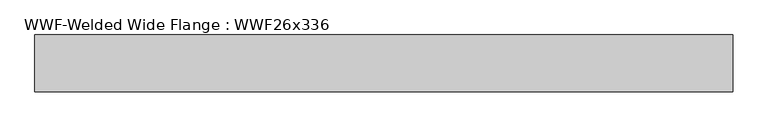
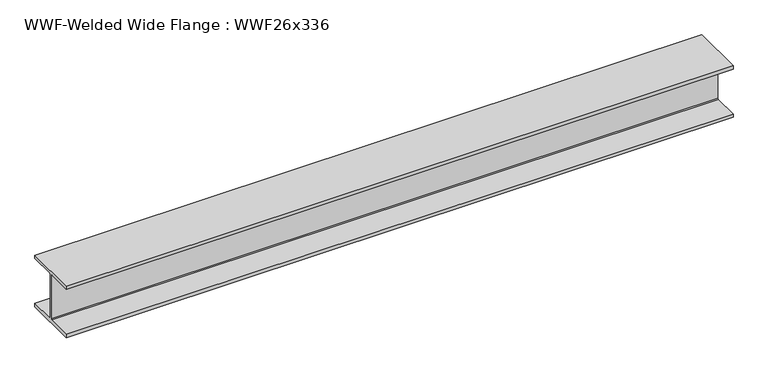
"""IFC4 building model written with IfcOpenShell, lengths in millimetres: beam geometry, WWF-Welded Wide Flange : WWF26x336."""

from ifc_helpers import new_model, si_unit, frame, origin, place, context, project, spatial, polyline, outline, extrude, source, transform, mapped, element, save


def wwf_welded_wide_flange_wwf26x336_27f69fbc(model_context):
    return source(origin(), model_context, "Body", "SweptSolid", [
        extrude(outline(polyline([(324.993, -284.988), (324.993, -324.993), (-324.993, -324.993), (-324.993, -284.988), (-20.6375, -284.988), (-9.9949, -274.3454), (-9.9949, 274.3454), (-20.6375, 284.988), (-324.993, 284.988), (-324.993, 324.993), (324.993, 324.993), (324.993, 284.988), (20.6375, 284.988), (9.9949, 274.3454), (9.9949, -274.3454), (20.6375, -284.988), (324.993, -284.988)])), frame((-3934.8877112, 0.0, 0.0), z_axis=(1.0, 0.0, 0.0), x_axis=(0.0, 1.0, 0.0)), (0.0, 0.0, 1.0), 7999.1189803),
    ])


if __name__ == "__main__":
    model = new_model("IFC4")
    model_context = context("Model", 3, world=origin())
    ifc_project = project(units=[si_unit("LENGTHUNIT", "METRE", prefix="MILLI")], contexts=[model_context])
    site = spatial("IfcSite", under=ifc_project)
    building = spatial("IfcBuilding", under=site)
    placement = place(None, origin())
    wwf_welded_wide_flange_wwf26x336_shape = wwf_welded_wide_flange_wwf26x336_27f69fbc(model_context)
    element("IfcBeam", 1, ObjectType="WWF-Welded Wide Flange : WWF26x336", at=placement, inside=building, context=model_context, shape_type="MappedRepresentation", body=[
        mapped(wwf_welded_wide_flange_wwf26x336_shape, transform((0.0, 0.0, 0.0), x_axis=(1.0, 0.0, 0.0), y_axis=(0.0, 1.0, 0.0), z_axis=(0.0, 0.0, 1.0))),
    ])
    save(model, "model.ifc")

# Revit data of these elements
# Type "WWF-Welded Wide Flange : WWF26x336"
#   Assembly Code = "B10"
#   Nominal d = "12"
#   W = 336
#   Length [instance default] = 1524 mm
#   bf = 649.986 mm
#   d = 649.986 mm
#   k = 20.638 mm
#   tf = 40.005 mm
#   tw = 19.99 mm
#   A = 0.0635483 m²
#   Structural Material [instance default] = Steel ASTM A572
# Element 1 (IfcBeam, "WWF-Welded Wide Flange : WWF26x336")
#   Structural Material = Metal - Steel 43-275
#   Materials on its faces: "Metal - Steel 43-275"
# Materials
#   "Steel ASTM A572": class "Metal", colour RGB 247 247 247, transparency 0, Description = "Structural steel, high strength low alloy, ASTM - A572 - 50", Cost = 0
#   "Metal - Steel 43-275": class "Metal", colour RGB 247 247 247, transparency 0, Cost = 0
